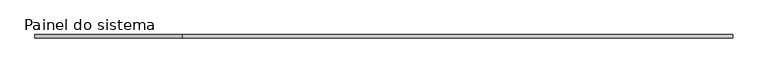
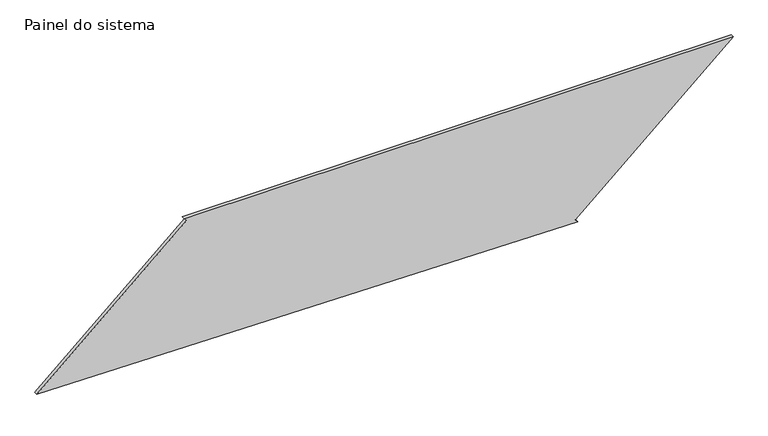
"""IFC4 building model written with IfcOpenShell, lengths in millimetres: plate geometry, Painel do sistema : Envidraçado."""

from ifc_helpers import new_model, si_unit, frame, origin, place, context, project, spatial, polyline, outline, extrude, source, transform, mapped, element, save


def painel_do_sistema_0c0ae910(model_context):
    return source(origin(), model_context, "Body", "SweptSolid", [
        extrude(outline(polyline([(0.0, 1358.2089488), (18.8079041, 1341.7388928), (992.3510691, 2453.472004), (992.3510691, -1413.5897561), (973.5431649, -1397.1197002), (48.4968973, -2453.472004), (0.0, 1358.2089488)])), frame((0.0, 24.5, 0.0), z_axis=(0.0, 1.0, 0.0), x_axis=(0.0, 0.0, 1.0)), (0.0, 0.0, 1.0), 25.0),
    ])


if __name__ == "__main__":
    model = new_model("IFC4")
    model_context = context("Model", 3, world=origin())
    ifc_project = project(units=[si_unit("LENGTHUNIT", "METRE", prefix="MILLI")], contexts=[model_context])
    site = spatial("IfcSite", under=ifc_project)
    building = spatial("IfcBuilding", under=site)
    placement = place(None, origin())
    painel_do_sistema_shape = painel_do_sistema_0c0ae910(model_context)
    element("IfcPlate", 1, ObjectType="Painel do sistema : Envidraçado", at=placement, inside=building, context=model_context, shape_type="MappedRepresentation", body=[
        mapped(painel_do_sistema_shape, transform((0.0, 0.0, 0.0), x_axis=(1.0, 0.0, 0.0), y_axis=(0.0, 1.0, 0.0), z_axis=(0.0, 0.0, 1.0))),
    ])
    save(model, "model.ifc")

# Revit data of these elements
# Type "Painel do sistema : Envidraçado"
#   Construction Type Id = "GSP4R"
#   Analytic Construction = "Vidraça única Pilkington 1/8 pol"
#   Visual Light Transmittance = 0.9
#   Solar Heat Gain Coefficient = 0.86
#   Heat Transfer Coefficient (U) = 6.7069 W/(m²·K)
# Element 1 (IfcPlate, "Painel do sistema : Envidraçado")
#   Materials on its faces: "Vidro"
# Materials
#   "Vidro": class "Vidro", colour RGB 0 128 192, transparency 0.9, Description = "Vidro de sílica", Cost = 0
